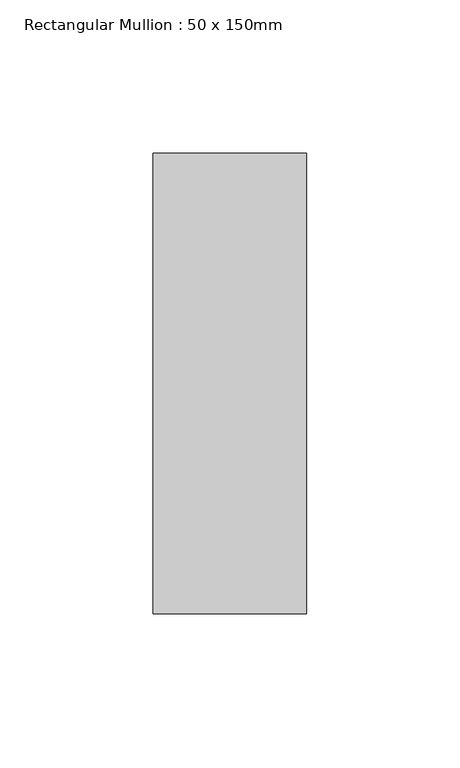
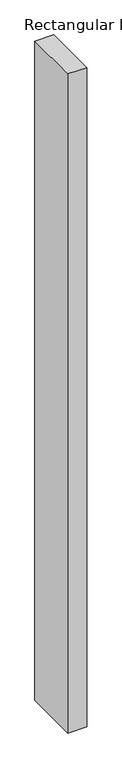
"""IFC4 building model written with IfcOpenShell, lengths in millimetres: member geometry, Rectangular Mullion : 50 x 150mm."""

from ifc_helpers import new_model, si_unit, frame, origin, place, context, project, spatial, polyline, outline, extrude, source, transform, mapped, element, save


def rectangular_mullion_50_x_150mm_43a70b30(model_context):
    return source(origin(), model_context, "Body", "SweptSolid", [
        extrude(outline(polyline([(0.0, 75.0), (0.0, -75.0), (-50.0, -75.0), (-50.0, 75.0), (0.0, 75.0)])), frame((0.0, 0.0, -1836.1666666), z_axis=(0.0, 0.0, 1.0), x_axis=(1.0, 0.0, 0.0)), (0.0, 0.0, 1.0), 1836.1666666),
    ])


if __name__ == "__main__":
    model = new_model("IFC4")
    model_context = context("Model", 3, world=origin())
    ifc_project = project(units=[si_unit("LENGTHUNIT", "METRE", prefix="MILLI")], contexts=[model_context])
    site = spatial("IfcSite", under=ifc_project)
    building = spatial("IfcBuilding", under=site)
    placement = place(None, origin())
    rectangular_mullion_50_x_150mm_shape = rectangular_mullion_50_x_150mm_43a70b30(model_context)
    element("IfcMember", 1, ObjectType="Rectangular Mullion : 50 x 150mm", at=placement, inside=building, context=model_context, shape_type="MappedRepresentation", body=[
        mapped(rectangular_mullion_50_x_150mm_shape, transform((0.0, 0.0, 0.0), x_axis=(1.0, 0.0, 0.0), y_axis=(0.0, 1.0, 0.0), z_axis=(0.0, 0.0, 1.0))),
    ])
    save(model, "model.ifc")

# Revit data of these elements
# Type "Rectangular Mullion : 50 x 150mm"
#   built-in parameter 1007304 = 0.492126 (stored number, unit not read)
#   built-in parameter 1007301 = 0.082021 (stored number, unit not read)
#   built-in parameter 1007300 = 0.082021 (stored number, unit not read)
# Element 1 (IfcMember, "Rectangular Mullion : 50 x 150mm")
#   Materials on its faces: "Metal - Aluminium"
# Materials
#   "Metal - Aluminium": class "Metal", colour RGB 247 247 247, transparency 0
